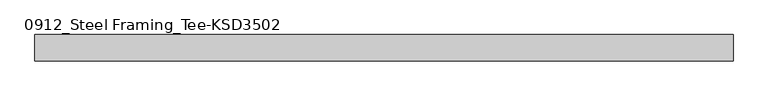
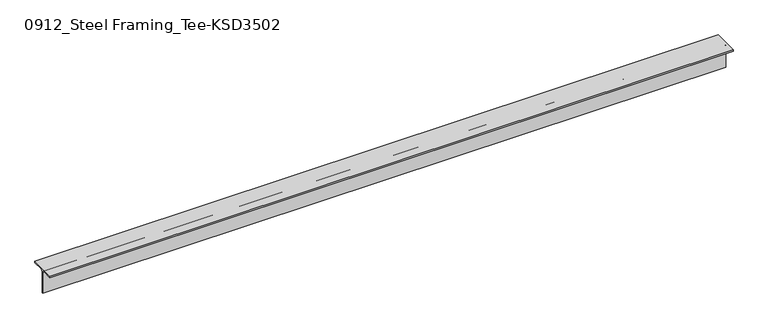
"""IFC4 building model written with IfcOpenShell, lengths in millimetres: member geometry, 0912_Steel Framing_Tee-KSD3502 : H_SB_ASB_CT-150x150x6.5x9."""

from ifc_helpers import new_model, si_unit, point, frame, frame_2d, origin, place, context, project, spatial, polyline, circle_curve, trimmed, segment, composite_curve, outline, extrude, source, transform, mapped, element, save


def member_0912_steel_framing_tee_ksd3502_c48fc55b(model_context):
    return source(origin(), model_context, "Body", "SweptSolid", [
        extrude(outline(composite_curve([segment(polyline([(75.0, 75.0), (75.0, 66.0), (16.25, 66.0)]), True, "CONTINUOUS"), segment(trimmed(circle_curve(frame_2d((16.25, 53.0)), 13.0), [point((16.25, 66.0))], [point((3.25, 53.0))], True, "CARTESIAN"), True, "CONTINUOUS"), segment(polyline([(3.25, 53.0), (3.25, -75.0), (-3.25, -75.0), (-3.25, 53.0)]), True, "CONTINUOUS"), segment(trimmed(circle_curve(frame_2d((-16.25, 53.0)), 13.0), [point((-3.25, 53.0))], [point((-16.25, 66.0))], True, "CARTESIAN"), True, "CONTINUOUS"), segment(polyline([(-16.25, 66.0), (-75.0, 66.0), (-75.0, 75.0), (75.0, 75.0)]), True, "CONTINUOUS")], self_intersect=False)), frame((-1979.35, 0.0, 0.0), z_axis=(1.0, 0.0, 0.0), x_axis=(0.0, 1.0, 0.0)), (0.0, 0.0, 1.0), 3944.8),
    ])


if __name__ == "__main__":
    model = new_model("IFC4")
    model_context = context("Model", 3, world=origin())
    ifc_project = project(units=[si_unit("LENGTHUNIT", "METRE", prefix="MILLI")], contexts=[model_context])
    site = spatial("IfcSite", under=ifc_project)
    building = spatial("IfcBuilding", under=site)
    placement = place(None, origin())
    member_0912_steel_framing_tee_ksd3502_shape = member_0912_steel_framing_tee_ksd3502_c48fc55b(model_context)
    element("IfcMember", 1, ObjectType="0912_Steel Framing_Tee-KSD3502 : H_SB_ASB_CT-150x150x6.5x9", at=placement, inside=building, context=model_context, shape_type="MappedRepresentation", body=[
        mapped(member_0912_steel_framing_tee_ksd3502_shape, transform((0.0, 0.0, 0.0), x_axis=(1.0, 0.0, 0.0), y_axis=(0.0, 1.0, 0.0), z_axis=(0.0, 0.0, 1.0))),
    ])
    save(model, "model.ifc")

# Revit data of these elements
# Type "0912_Steel Framing_Tee-KSD3502 : H_SB_ASB_CT-150x150x6.5x9"
#   H_WM Code_1 = "S01AA003-00001 | Main Steel Structure Fabrication Work | Shelter/Building | Light Steel - Standard (30KG/M>Weight) | Material: (   )"
#   H_WM Code_2 = "S03AA029-00001 | Main Steel Structure Erection Work | Shelter/Building | Light Steel (30KG/M>Weight) | Material: (   )"
#   H_WM Code_3 = "S01AA010-00001 | Main Steel Structure Fabrication Work | Shelter/Building | Steel Painting/Coating | for Non-Fireproofed Steel Surface, Surface Preparation, Primer, Second & Final Coat | Material: (   )"
#   H_Q'ty Cal Type Tag = "SB-Q2"
#   Width = 15.0 cm
#   Web Thickness = 0.65 cm
#   Web Fillet = 1.3 cm
#   Section Area = 23.39 cm²
#   Perimeter = 0.60 m²/m
#   Nominal Weight = 18.40 kgf/m
#   Height = 15.0 cm
#   Flange Thickness = 0.9 cm
#   Centroid Vertical = 7.5 cm
#   Centroid Horizontal = 7.5 cm
#   Length [instance default] = 1.5000 m
#   Structural Material [instance default] = Steel, 45-345
#   Warping Constant = (empty or 0)
#   Torsional Moment of Inertia = 0
#   Section Name Key = ""
#   Plastic Modulus weak axis = 0
#   Plastic Modulus strong axis = 0
#   Moment of Inertia weak axis = 0
#   Moment of Inertia strong axis = 0
#   Elastic Modulus weak axis = 0
#   Elastic Modulus strong axis = 0
#   Bolt Spacing = 0
#   Assembly Code = ""
# Element 1 (IfcMember, "0912_Steel Framing_Tee-KSD3502 : H_SB_ASB_CT-150x150x6.5x9")
#   Structural Material = none
# Materials
#   "Steel, 45-345": class "Metal", colour RGB 189 187 185, transparency 0, Description = "Steel 345 MPa", Cost = 0
